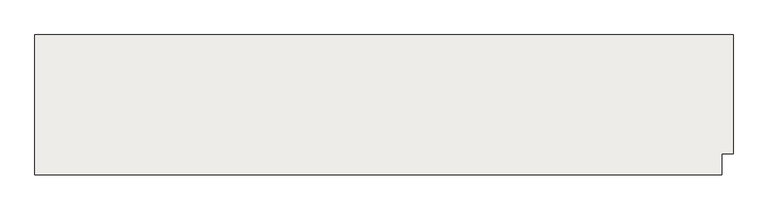
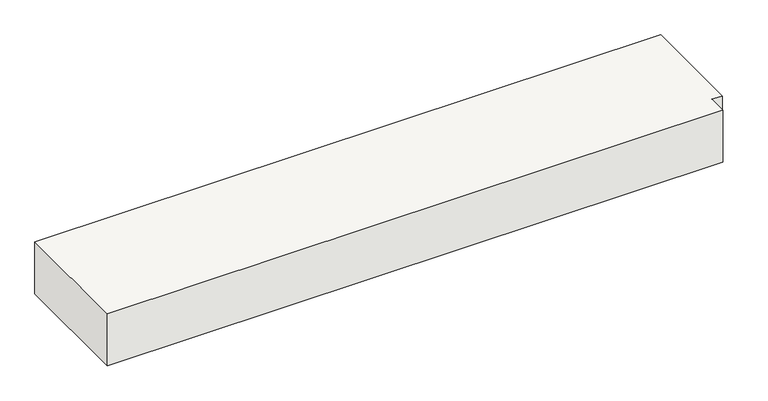
"""IFC4 building model written with IfcOpenShell, lengths in millimetres: slab geometry, Pano 22 (16 cm)."""

from ifc_helpers import new_model, si_unit, origin, origin_with_axes, place, context, project, spatial, polyline, outline, extrude, source, transform, mapped, element, save


def slab_97b672c3(model_context):
    return source(origin(), model_context, "Body", "SweptSolid", [
        extrude(outline(polyline([(3940.0, 10495.0), (3940.0, 10860.09152), (5760.0, 10860.11594), (5760.0, 10550.0), (5730.0, 10550.0), (5730.0, 10495.0), (3940.0, 10495.0)])), origin_with_axes(), (0.0, 0.0, 1.0), 160.0),
    ])


if __name__ == "__main__":
    model = new_model("IFC4")
    model_context = context("Model", 3, world=origin())
    ifc_project = project(units=[si_unit("LENGTHUNIT", "METRE", prefix="MILLI")], contexts=[model_context])
    site = spatial("IfcSite", under=ifc_project)
    building = spatial("IfcBuilding", under=site)
    placement = place(None, origin())
    slab_shape = slab_97b672c3(model_context)
    element("IfcSlab", 1, ObjectType="Pano 22 (16 cm)", at=placement, inside=building, context=model_context, shape_type="MappedRepresentation", body=[
        mapped(slab_shape, transform((0.0, 0.0, 0.0), x_axis=(1.0, 0.0, 0.0), y_axis=(0.0, 1.0, 0.0), z_axis=(0.0, 0.0, 1.0))),
    ])
    save(model, "model.ifc")

# Revit data of these elements
# Element 1 (IfcSlab, "Pano 22 (16 cm)")
#   Materials on its faces: "RGB 168-169-158"
# Materials
#   "RGB 168-169-158": class "Não atribuído", colour RGB 168 169 158, transparency 0
